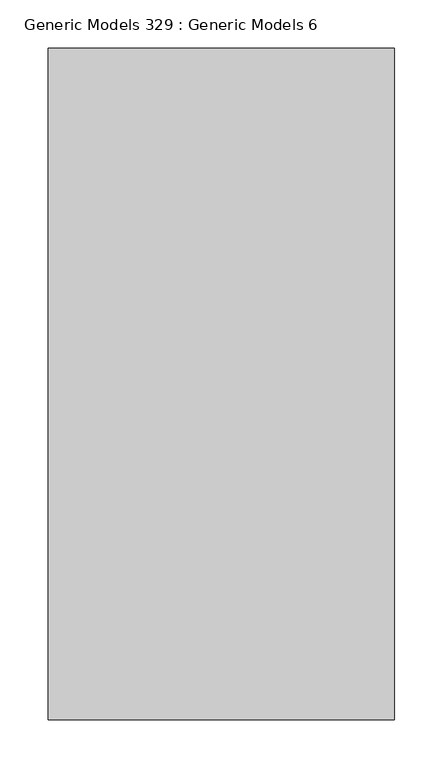
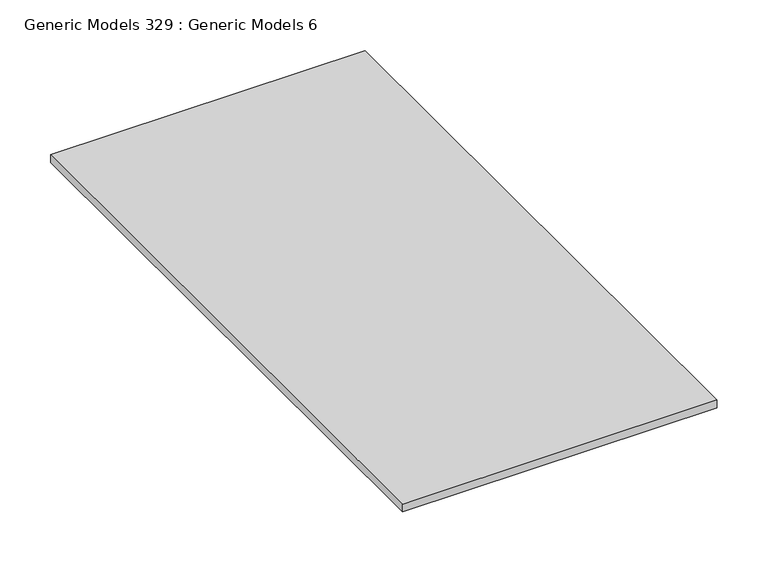
"""IFC4 building model written with IfcOpenShell, lengths in millimetres: proxy geometry, Generic Models 329 : Generic Models 6."""

from ifc_helpers import new_model, si_unit, frame, origin, place, context, project, spatial, polyline, outline, extrude, source, transform, mapped, element, save


def generic_models_329_generic_models_6_de1754a4(model_context):
    return source(origin(), model_context, "Body", "SweptSolid", [
        extrude(outline(polyline([(1257.1263704, 1781.5884092), (1616.549618, 1781.5884092), (1616.549618, 1085.5309662), (1257.1263704, 1085.5309662), (1257.1263704, 1781.5884092)])), frame((0.0, 0.0, 123459.621), z_axis=(0.0, 0.0, 1.0), x_axis=(1.0, 0.0, 0.0)), (0.0, 0.0, 1.0), 9.525),
    ])


if __name__ == "__main__":
    model = new_model("IFC4")
    model_context = context("Model", 3, world=origin())
    ifc_project = project(units=[si_unit("LENGTHUNIT", "METRE", prefix="MILLI")], contexts=[model_context])
    site = spatial("IfcSite", under=ifc_project)
    building = spatial("IfcBuilding", under=site)
    placement = place(None, origin())
    generic_models_329_generic_models_6_shape = generic_models_329_generic_models_6_de1754a4(model_context)
    element("IfcBuildingElementProxy", 1, Name="Generic Models 329 : Generic Models 6", ObjectType="Generic Models 329 : Generic Models 6", at=placement, inside=building, context=model_context, shape_type="MappedRepresentation", body=[
        mapped(generic_models_329_generic_models_6_shape, transform((0.0, 0.0, 0.0), x_axis=(1.0, 0.0, 0.0), y_axis=(0.0, 1.0, 0.0), z_axis=(0.0, 0.0, 1.0))),
    ])
    save(model, "model.ifc")

# Revit data of these elements
# Element 1 (IfcBuildingElementProxy, "Generic Models 329 : Generic Models 6")
#   Materials on its faces: "_STONE TILE - T.B.D."
# Materials
#   "_STONE TILE - T.B.D.": class "Generic", colour RGB 233 233 233, transparency 0, Cost = 0
